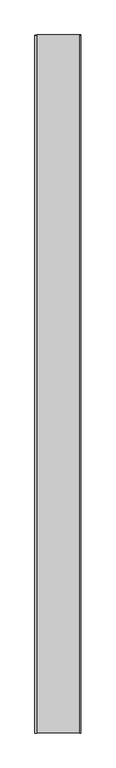
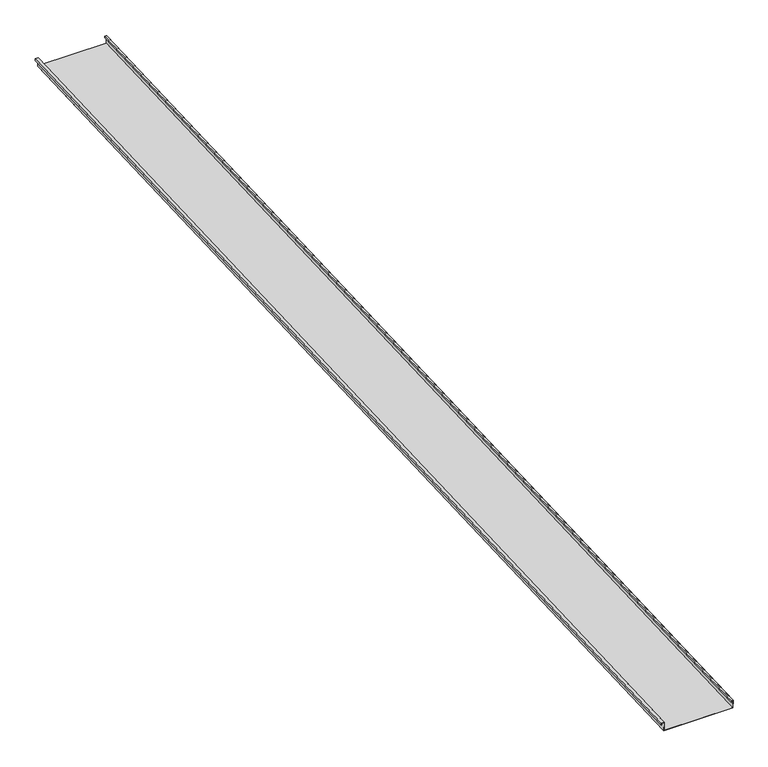
"""IFC4 building model written with IfcOpenShell, lengths in millimetres: proxy geometry, Generic Models 2:Generic Models 2:310765:Generic Models 2:310765 : Generic Models 2:Generic Models 2:310765:120 : Generic Models 2:Generic Models 2:310765:Generic Models 2:310765 : Generic Models 2:Generic Models 2:310765:300385."""

from ifc_helpers import new_model, si_unit, frame, origin, place, context, project, spatial, polyline, outline, extrude, source, transform, mapped, element, save


def generic_models_8ccb9adb(model_context):
    return source(origin(), model_context, "Body", "SweptSolid", [
        extrude(outline(polyline([(1.5875, 0.0), (1.5875, 50.8), (407.9875, 50.8), (407.9875, 1.5875), (396.875, 1.5875), (396.875, 11.1125), (398.4625, 11.1125), (398.4625, 3.175), (406.4, 3.175), (406.4, 49.2125), (3.175, 49.2125), (3.175, -1.5874999), (-14.2875, -1.5874999), (-14.2875, 9.525), (-12.7, 9.525), (-12.7, 0.0), (1.5875, 0.0)])), frame((663801.0763072, -581354.4345603, 3902.6697972), z_axis=(0.0, 0.9991330730923568, 0.041630544712067834), x_axis=(1.0, 0.0, 0.0)), (0.0, 0.0, 1.0), 6400.8),
    ])


if __name__ == "__main__":
    model = new_model("IFC4")
    model_context = context("Model", 3, world=origin())
    ifc_project = project(units=[si_unit("LENGTHUNIT", "METRE", prefix="MILLI")], contexts=[model_context])
    site = spatial("IfcSite", under=ifc_project)
    building = spatial("IfcBuilding", under=site)
    placement = place(None, origin())
    generic_models_shape = generic_models_8ccb9adb(model_context)
    element("IfcBuildingElementProxy", 1, Name="Generic Models 2:Generic Models 2:310765:Generic Models 2:310765 : Generic Models 2:Generic Models 2:310765:120 : Generic Models 2:Generic Models 2:310765:Generic Models 2:310765 : Generic Models 2:Generic Models 2:310765:300385", ObjectType="Generic Models 2:Generic Models 2:310765:Generic Models 2:310765 : Generic Models 2:Generic Models 2:310765:120 : Generic Models 2:Generic Models 2:310765:Generic Models 2:310765 : Generic Models 2:Generic Models 2:310765:300385", at=placement, inside=building, context=model_context, shape_type="MappedRepresentation", body=[
        mapped(generic_models_shape, transform((0.0, 0.0, 0.0), x_axis=(1.0, 0.0, 0.0), y_axis=(0.0, 1.0, 0.0), z_axis=(0.0, 0.0, 1.0))),
    ])
    save(model, "model.ifc")

# Revit data of these elements
# Type "Generic Models 2:Generic Models 2:310765:Generic Models 2:310765 : Generic Models 2:Generic Models 2:310765:120 : Generic Models 2:Generic Models 2:310765:Generic Models 2:310765 : Generic Models 2:Generic Models 2:310765:300385"
#   NameOverride = "Generic Models 2:Generic Models 2:310765:Generic Models 2:310765 : Generic Models 2:Generic Models 2:310765:300385"
#   ObjectTypeOverride = "Generic Models 2:310765 : Generic Models 2:Generic Models 2:310765"
#   Reference = "Generic Models 2"
#   Tag = "300385"
# Element 1 (IfcBuildingElementProxy, "Generic Models 2:Generic Models 2:310765:Generic Models 2:310765 : Generic Models 2:Generic Models 2:310765:120 : Generic Models 2:Generic Models 2:310765:Generic Models 2:310765 : Generic Models 2:Generic Models 2:310765:300385")
#   Materials on its faces: "THERMAL BROKEN ALUMINUM STOREFRONT FOR POLYCARBONATE"
# Materials
#   "THERMAL BROKEN ALUMINUM STOREFRONT FOR POLYCARBONATE": class "Unassigned", colour RGB 244 244 244, transparency 0, Keynote = "M07611300.01", Cost = 0
